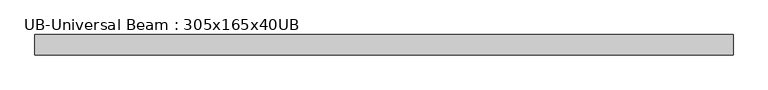
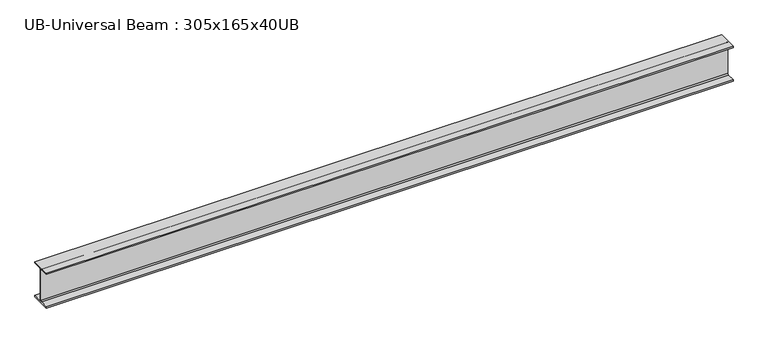
"""IFC4 building model written with IfcOpenShell, lengths in millimetres: beam geometry, UB-Universal Beam : 305x165x40UB."""

from ifc_helpers import new_model, si_unit, point, frame, frame_2d, origin, place, context, project, spatial, polyline, circle_curve, trimmed, segment, composite_curve, outline, extrude, source, transform, mapped, element, save


def ub_universal_beam_305x165x40ub_9b2e80cd(model_context):
    return source(origin(), model_context, "Body", "SweptSolid", [
        extrude(outline(composite_curve([segment(polyline([(82.5, -141.5), (82.5, -151.7), (-82.5, -151.7), (-82.5, -141.5), (-11.9, -141.5)]), True, "CONTINUOUS"), segment(trimmed(circle_curve(frame_2d((-11.9, -132.6)), 8.9), [point((-11.9, -141.5))], [point((-3.0, -132.6))], True, "CARTESIAN"), True, "CONTINUOUS"), segment(polyline([(-3.0, -132.6), (-3.0, 132.6)]), True, "CONTINUOUS"), segment(trimmed(circle_curve(frame_2d((-11.9, 132.6)), 8.9), [point((-3.0, 132.6))], [point((-11.9, 141.5))], True, "CARTESIAN"), True, "CONTINUOUS"), segment(polyline([(-11.9, 141.5), (-82.5, 141.5), (-82.5, 151.7), (82.5, 151.7), (82.5, 141.5), (11.9, 141.5)]), True, "CONTINUOUS"), segment(trimmed(circle_curve(frame_2d((11.9, 132.6)), 8.9), [point((11.9, 141.5))], [point((3.0, 132.6))], True, "CARTESIAN"), True, "CONTINUOUS"), segment(polyline([(3.0, 132.6), (3.0, -132.6)]), True, "CONTINUOUS"), segment(trimmed(circle_curve(frame_2d((11.9, -132.6)), 8.9), [point((3.0, -132.6))], [point((11.9, -141.5))], True, "CARTESIAN"), True, "CONTINUOUS"), segment(polyline([(11.9, -141.5), (82.5, -141.5)]), True, "CONTINUOUS")], self_intersect=False)), frame((-2834.65, 0.0, 0.0), z_axis=(1.0, 0.0, 0.0), x_axis=(0.0, 1.0, 0.0)), (0.0, 0.0, 1.0), 5668.0),
    ])


if __name__ == "__main__":
    model = new_model("IFC4")
    model_context = context("Model", 3, world=origin())
    ifc_project = project(units=[si_unit("LENGTHUNIT", "METRE", prefix="MILLI")], contexts=[model_context])
    site = spatial("IfcSite", under=ifc_project)
    building = spatial("IfcBuilding", under=site)
    placement = place(None, origin())
    ub_universal_beam_305x165x40ub_shape = ub_universal_beam_305x165x40ub_9b2e80cd(model_context)
    element("IfcBeam", 1, ObjectType="UB-Universal Beam : 305x165x40UB", at=placement, inside=building, context=model_context, shape_type="MappedRepresentation", body=[
        mapped(ub_universal_beam_305x165x40ub_shape, transform((0.0, 0.0, 0.0), x_axis=(1.0, 0.0, 0.0), y_axis=(0.0, 1.0, 0.0), z_axis=(0.0, 0.0, 1.0))),
    ])
    save(model, "model.ifc")

# Revit data of these elements
# Type "UB-Universal Beam : 305x165x40UB"
#   Nominal h = "305"
#   W = 0
#   Start Extension Calculation [instance default] = 3000 mm
#   Start Extension [instance default] = -12.7 mm
#   End Extension Calculation [instance default] = 3000 mm
#   End Extension [instance default] = -12.7 mm
#   Ix = 8503
#   Length [instance default] = 1524 mm
#   M = 40.3
#   Zx = 560
#   b = 165 mm
#   h = 303.4 mm
#   r = 8.9 mm
#   s = 6 mm
#   t = 10.2 mm
#   A = 0.005 m²
#   Structural Material [instance default] = Metal - Steel - 345 MPa
#   Assembly Code = ""
# Element 1 (IfcBeam, "UB-Universal Beam : 305x165x40UB")
#   Materials on its faces: "Metal - Steel - 345 MPa"
# Materials
#   "Metal - Steel - 345 MPa": class "Metal", colour RGB 241 46 46, transparency 0
